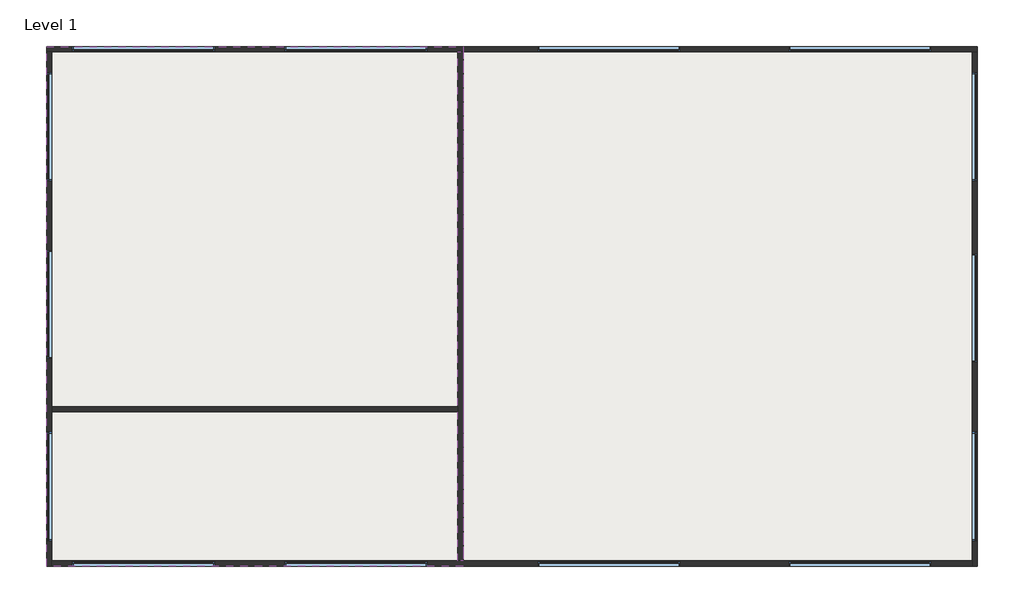
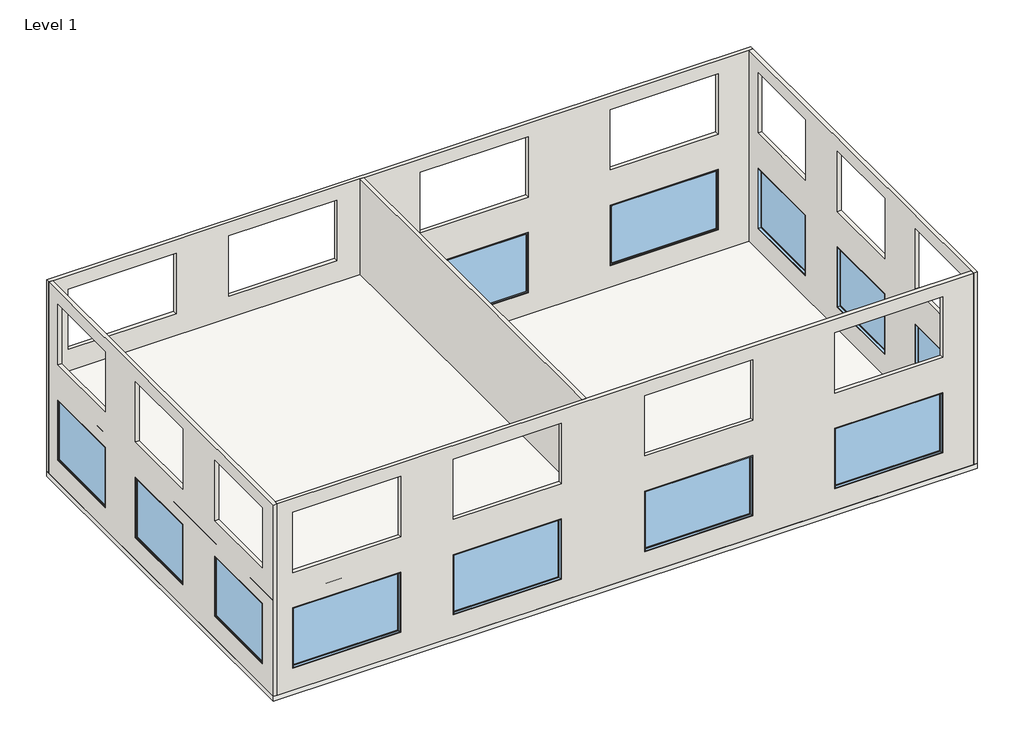
# One storey: 14 windows, 7 walls, 2 slabs.
"""IFC4 building model written with IfcOpenShell, lengths in millimetres."""

import ifcopenshell
import ifcopenshell.guid

model = None  # the IFC model being written
_history = None  # IfcOwnerHistory: only IFC2X3 demands one
_inside = {}  # id of a spatial element -> (the spatial element, [elements in it])
_under = {}  # id of a project, library or spatial element -> (it, [spatial elements below it])
_declared = {}  # id of a project -> (the project, [libraries it declares])
_typed = {}  # id of a type object -> (the type object, [elements of that type])
_made_of = {}  # id of a material, layer set ... -> (it, [elements and type objects made of it])


def new_model(schema):
    """Start an empty IFC model of exactly this schema.

    Asked for "IFC4X3", IfcOpenShell would pick the latest addendum, in which some entities
    have other attributes; the version numbers below select the first issue.
    IFC2X3 requires an IfcOwnerHistory on every rooted entity: one is made here for all.
    """
    global model, _history
    if schema == "IFC4X3":
        model = ifcopenshell.file(schema_version=(4, 3, 0, 0))
    else:
        model = ifcopenshell.file(schema=schema)
    _inside.clear()
    _under.clear()
    _declared.clear()
    _typed.clear()
    _made_of.clear()
    _history = None
    if model.schema == "IFC2X3":
        org = make("IfcOrganization", Name="unknown")
        user = make(
            "IfcPersonAndOrganization",
            ThePerson=make("IfcPerson", FamilyName="unknown"),
            TheOrganization=org,
        )
        app = make(
            "IfcApplication",
            ApplicationDeveloper=org,
            Version="unknown",
            ApplicationFullName="unknown",
            ApplicationIdentifier="unknown",
        )
        _history = make(
            "IfcOwnerHistory",
            OwningUser=user,
            OwningApplication=app,
            ChangeAction="ADDED",
            CreationDate=0,
        )
    return model


def make(cls, **values):
    """One entity of the class cls with the attributes given. An attribute that is None is left unset."""
    return model.create_entity(
        cls, **{name: value for name, value in values.items() if value is not None}
    )


def rooted(cls, **values):
    """An entity with a GlobalId (a new one), such as an element, a storey or a relation."""
    return make(cls, GlobalId=ifcopenshell.guid.new(), OwnerHistory=_history, **values)


def si_unit(unit_type, name, prefix=None):
    """IfcSIUnit, for example si_unit("LENGTHUNIT", "METRE", prefix="MILLI")."""
    return make("IfcSIUnit", UnitType=unit_type, Prefix=prefix, Name=name)


def assignment(units):
    """IfcUnitAssignment: the units of a project."""
    return None if units is None else make("IfcUnitAssignment", Units=units)


def point(xyz):
    """IfcCartesianPoint."""
    return None if xyz is None else make("IfcCartesianPoint", Coordinates=xyz)


def direction(xyz):
    """IfcDirection."""
    return None if xyz is None else make("IfcDirection", DirectionRatios=xyz)


def frame(location, z_axis=None, x_axis=None):
    """IfcAxis2Placement3D, a coordinate frame: its origin and axes. An axis left out is left unset."""
    return make(
        "IfcAxis2Placement3D",
        Location=point(location),
        Axis=direction(z_axis),
        RefDirection=direction(x_axis),
    )


def origin():
    """The frame at (0, 0, 0) with its axes left unset."""
    return frame((0.0, 0.0, 0.0))


def origin_with_axes():
    """The frame at (0, 0, 0) with the z axis (0, 0, 1) and the x axis (1, 0, 0) written out."""
    return frame((0.0, 0.0, 0.0), z_axis=(0.0, 0.0, 1.0), x_axis=(1.0, 0.0, 0.0))


def place(relative_to, where):
    """IfcLocalPlacement: puts the frame where relative to a parent placement (None: the world)."""
    return make(
        "IfcLocalPlacement", PlacementRelTo=relative_to, RelativePlacement=where
    )


def context(
    kind, dimensions, precision=None, world=None, true_north=None, identifier=None
):
    """IfcGeometricRepresentationContext, for example the 3D "Model" context."""
    return make(
        "IfcGeometricRepresentationContext",
        ContextIdentifier=identifier,
        ContextType=kind,
        CoordinateSpaceDimension=dimensions,
        Precision=precision,
        WorldCoordinateSystem=world,
        TrueNorth=true_north,
    )


def project(units=None, contexts=None):
    """IfcProject with its units and contexts."""
    return rooted(
        "IfcProject",
        Name="project",
        RepresentationContexts=contexts,
        UnitsInContext=assignment(units),
    )


def spatial(cls, under=None, at=None, **own):
    """A site, building, storey or space (cls), placed at a placement, below another one or the project."""
    s = rooted(cls, ObjectPlacement=at, **own)
    if under is not None:
        _under.setdefault(under.id(), (under, []))[1].append(s)
    return s


def polyline(points):
    """IfcPolyline through the points."""
    return make("IfcPolyline", Points=[point(p) for p in points])


def outline(outer, holes=None, kind="AREA"):
    """IfcArbitraryClosedProfileDef: a profile drawn as a closed curve; with holes, ...WithVoids."""
    if holes is None:
        return make("IfcArbitraryClosedProfileDef", ProfileType=kind, OuterCurve=outer)
    return make(
        "IfcArbitraryProfileDefWithVoids",
        ProfileType=kind,
        OuterCurve=outer,
        InnerCurves=holes,
    )


def extrude(swept, where, along, depth):
    """IfcExtrudedAreaSolid: the profile swept, set in the frame where, extruded along a direction by depth."""
    return make(
        "IfcExtrudedAreaSolid",
        SweptArea=swept,
        Position=where,
        ExtrudedDirection=direction(along),
        Depth=depth,
    )


def faces_of(points, faces, orient=None, outer=None):
    """IfcFace entities. A face is a list of loops; a loop is a list of indices into points, from 0.

    orient and outer hold one flag for each loop. By default every Orientation is true, the
    first loop of a face is its IfcFaceOuterBound and the others are IfcFaceBound.
    """
    made = []
    for i, loops in enumerate(faces):
        bounds = []
        for j, loop in enumerate(loops):
            is_outer = j == 0 if outer is None else outer[i][j]
            bounds.append(
                make(
                    "IfcFaceOuterBound" if is_outer else "IfcFaceBound",
                    Bound=make("IfcPolyLoop", Polygon=[points[k] for k in loop]),
                    Orientation=True if orient is None else orient[i][j],
                )
            )
        made.append(make("IfcFace", Bounds=bounds))
    return made


def faceted_brep(points, faces, orient=None, outer=None, voids=None):
    """IfcFacetedBrep: a solid bounded by flat faces; with voids (closed shells), ...WithVoids."""
    shared = [point(p) for p in points]
    hull = make("IfcClosedShell", CfsFaces=faces_of(shared, faces, orient, outer))
    if voids is None:
        return make("IfcFacetedBrep", Outer=hull)
    return make(
        "IfcFacetedBrepWithVoids",
        Outer=hull,
        Voids=[
            make(cls, CfsFaces=faces_of(shared, fs, o, b)) for cls, fs, o, b in voids
        ],
    )


def shape(context_of_items, identifier, shape_type, items):
    """IfcShapeRepresentation: the items that make up one representation, for example the "Body"."""
    return make(
        "IfcShapeRepresentation",
        ContextOfItems=context_of_items,
        RepresentationIdentifier=identifier,
        RepresentationType=shape_type,
        Items=items,
    )


def source(mapping_origin, context_of_items, identifier, shape_type, items):
    """IfcRepresentationMap: a shape defined once, which mapped items show again and again."""
    return make(
        "IfcRepresentationMap",
        MappingOrigin=mapping_origin,
        MappedRepresentation=shape(context_of_items, identifier, shape_type, items),
    )


def transform(
    local_origin,
    x_axis=None,
    y_axis=None,
    z_axis=None,
    scale=None,
    scale2=None,
    scale3=None,
    uniform=True,
):
    """IfcCartesianTransformationOperator3D, or its non-uniform kind. x_axis, y_axis, z_axis: its Axis1, 2, 3."""
    if uniform:
        return make(
            "IfcCartesianTransformationOperator3D",
            Axis1=direction(x_axis),
            Axis2=direction(y_axis),
            LocalOrigin=point(local_origin),
            Scale=scale,
            Axis3=direction(z_axis),
        )
    return make(
        "IfcCartesianTransformationOperator3DnonUniform",
        Axis1=direction(x_axis),
        Axis2=direction(y_axis),
        LocalOrigin=point(local_origin),
        Scale=scale,
        Axis3=direction(z_axis),
        Scale2=scale2,
        Scale3=scale3,
    )


def mapped(mapping_source, mapping_target):
    """IfcMappedItem: shows the shape of a source again, moved by a transform."""
    return make(
        "IfcMappedItem", MappingSource=mapping_source, MappingTarget=mapping_target
    )


def made_of(thing, what):
    """Note that an element or type object is made of a material, layer set ...; save() writes the relation."""
    if what is not None:
        _made_of.setdefault(what.id(), (what, []))[1].append(thing)
    return thing


def element(
    cls,
    number,
    at=None,
    inside=None,
    cuts=None,
    type_object=None,
    material=None,
    context=None,
    identifier="Body",
    shape_type=None,
    held_by="IfcProductDefinitionShape",
    body=None,
    shapes=None,
    **own,
):
    """One element of the class cls, such as IfcWall. Its Tag is "e" and its number.

    at: its placement. inside: the storey or other place that contains it. cuts: it is an
    opening in that element (IfcRelVoidsElement). A single representation is given by context,
    identifier, shape_type and body (its items); several are given by shapes. held_by: the class
    of the entity that holds the representations. save() writes the other relations.
    """
    e = rooted(cls, Tag="e%d" % number, ObjectPlacement=at, **own)
    if body is not None:
        shapes = [shape(context, identifier, shape_type, body)]
    if shapes is not None:
        e.Representation = make(held_by, Representations=shapes)
    if inside is not None:
        _inside.setdefault(inside.id(), (inside, []))[1].append(e)
    if cuts is not None:
        rooted(
            "IfcRelVoidsElement", RelatingBuildingElement=cuts, RelatedOpeningElement=e
        )
    if type_object is not None:
        _typed.setdefault(type_object.id(), (type_object, []))[1].append(e)
    return made_of(e, material)


def aggregate(whole, parts):
    """IfcRelAggregates: a whole, such as a stair, and the parts it consists of."""
    return rooted("IfcRelAggregates", RelatingObject=whole, RelatedObjects=parts)


def save(model, path):
    """Write the relations noted so far, then the file.

    IfcRelAggregates (storeys below a building ...), IfcRelContainedInSpatialStructure (elements
    in a storey), IfcRelDefinesByType, IfcRelAssociatesMaterial and IfcRelDeclares: one each for
    every whole, place, type object, material and project.
    """
    for whole, parts in _under.values():
        aggregate(whole, parts)
    for where, things in _inside.values():
        rooted(
            "IfcRelContainedInSpatialStructure",
            RelatedElements=things,
            RelatingStructure=where,
        )
    for kind, things in _typed.values():
        rooted("IfcRelDefinesByType", RelatedObjects=things, RelatingType=kind)
    for what, things in _made_of.values():
        rooted("IfcRelAssociatesMaterial", RelatedObjects=things, RelatingMaterial=what)
    for by, libraries in _declared.values():
        rooted("IfcRelDeclares", RelatingContext=by, RelatedDefinitions=libraries)
    model.write(path)


def m_fixed_2500x_4228mm_fd5e51e7(model_context):
    return source(origin(), model_context, "Body", "SweptSolid", [
        extrude(outline(polyline([(-2050.8, 54.2), (2050.8, 54.2), (2050.8, 42.2), (-2050.8, 42.2), (-2050.8, 54.2)])), frame((0.0, 0.0, 368.0), z_axis=(0.0, 0.0, 1.0), x_axis=(1.0, 0.0, 0.0)), (0.0, 0.0, 1.0), 2374.0),
        extrude(outline(polyline([(2786.0, -2094.8), (324.0, -2094.8), (324.0, 2094.8), (2786.0, 2094.8), (2786.0, -2094.8)]), holes=[polyline([(2742.0, -2050.8), (2742.0, 2050.8), (368.0, 2050.8), (368.0, -2050.8), (2742.0, -2050.8)])]), frame((0.0, 26.2, 0.0), z_axis=(0.0, 1.0, 0.0), x_axis=(0.0, 0.0, 1.0)), (0.0, 0.0, 1.0), 44.0),
        extrude(outline(polyline([(2805.0, -2113.8), (305.0, -2113.8), (305.0, 2113.8), (2805.0, 2113.8), (2805.0, -2113.8)]), holes=[polyline([(2786.0, -2094.8), (2786.0, 2094.8), (324.0, 2094.8), (324.0, -2094.8), (2786.0, -2094.8)])]), frame((0.0, 26.2, 0.0), z_axis=(0.0, 1.0, 0.0), x_axis=(0.0, 0.0, 1.0)), (0.0, 0.0, 1.0), 63.0),
        extrude(outline(polyline([(2805.0, -2113.8), (305.0, -2113.8), (305.0, 2113.8), (2805.0, 2113.8), (2805.0, -2113.8)]), holes=[polyline([(2773.0, -2081.8), (2773.0, 2081.8), (337.0, 2081.8), (337.0, -2081.8), (2773.0, -2081.8)])]), frame((0.0, -63.2, 0.0), z_axis=(0.0, 1.0, 0.0), x_axis=(0.0, 0.0, 1.0)), (0.0, 0.0, 1.0), 89.4),
    ])


def m_fixed_2500x_4228mm_f14c179f(model_context):
    return source(origin(), model_context, "Body", "SweptSolid", [
        extrude(outline(polyline([(-2050.8, -54.2), (-2050.8, -42.2), (2050.8, -42.2), (2050.8, -54.2), (-2050.8, -54.2)])), frame((0.0, 0.0, 368.0), z_axis=(0.0, 0.0, 1.0), x_axis=(1.0, 0.0, 0.0)), (0.0, 0.0, 1.0), 2374.0),
        extrude(outline(polyline([(2786.0, -2094.8), (324.0, -2094.8), (324.0, 2094.8), (2786.0, 2094.8), (2786.0, -2094.8)]), holes=[polyline([(2742.0, -2050.8), (2742.0, 2050.8), (368.0, 2050.8), (368.0, -2050.8), (2742.0, -2050.8)])]), frame((0.0, -70.2, 0.0), z_axis=(0.0, 1.0, 0.0), x_axis=(0.0, 0.0, 1.0)), (0.0, 0.0, 1.0), 44.0),
        extrude(outline(polyline([(2805.0, -2113.8), (305.0, -2113.8), (305.0, 2113.8), (2805.0, 2113.8), (2805.0, -2113.8)]), holes=[polyline([(2786.0, -2094.8), (2786.0, 2094.8), (324.0, 2094.8), (324.0, -2094.8), (2786.0, -2094.8)])]), frame((0.0, -89.2, 0.0), z_axis=(0.0, 1.0, 0.0), x_axis=(0.0, 0.0, 1.0)), (0.0, 0.0, 1.0), 63.0),
        extrude(outline(polyline([(2805.0, -2113.8), (305.0, -2113.8), (305.0, 2113.8), (2805.0, 2113.8), (2805.0, -2113.8)]), holes=[polyline([(2773.0, -2081.8), (2773.0, 2081.8), (337.0, 2081.8), (337.0, -2081.8), (2773.0, -2081.8)])]), frame((0.0, -26.2, 0.0), z_axis=(0.0, 1.0, 0.0), x_axis=(0.0, 0.0, 1.0)), (0.0, 0.0, 1.0), 89.4),
    ])


def m_fixed_2500x_3220mm_df94f4d0(model_context):
    return source(origin(), model_context, "Body", "SweptSolid", [
        extrude(outline(polyline([(-1546.8, 54.2), (1546.8, 54.2), (1546.8, 42.2), (-1546.8, 42.2), (-1546.8, 54.2)])), frame((0.0, 0.0, 368.0), z_axis=(0.0, 0.0, 1.0), x_axis=(1.0, 0.0, 0.0)), (0.0, 0.0, 1.0), 2374.0),
        extrude(outline(polyline([(2786.0, -1590.8), (324.0, -1590.8), (324.0, 1590.8), (2786.0, 1590.8), (2786.0, -1590.8)]), holes=[polyline([(2742.0, -1546.8), (2742.0, 1546.8), (368.0, 1546.8), (368.0, -1546.8), (2742.0, -1546.8)])]), frame((0.0, 26.2, 0.0), z_axis=(0.0, 1.0, 0.0), x_axis=(0.0, 0.0, 1.0)), (0.0, 0.0, 1.0), 44.0),
        extrude(outline(polyline([(2805.0, -1609.8), (305.0, -1609.8), (305.0, 1609.8), (2805.0, 1609.8), (2805.0, -1609.8)]), holes=[polyline([(2786.0, -1590.8), (2786.0, 1590.8), (324.0, 1590.8), (324.0, -1590.8), (2786.0, -1590.8)])]), frame((0.0, 26.2, 0.0), z_axis=(0.0, 1.0, 0.0), x_axis=(0.0, 0.0, 1.0)), (0.0, 0.0, 1.0), 63.0),
        extrude(outline(polyline([(2805.0, -1609.8), (305.0, -1609.8), (305.0, 1609.8), (2805.0, 1609.8), (2805.0, -1609.8)]), holes=[polyline([(2773.0, -1577.8), (2773.0, 1577.8), (337.0, 1577.8), (337.0, -1577.8), (2773.0, -1577.8)])]), frame((0.0, -63.2, 0.0), z_axis=(0.0, 1.0, 0.0), x_axis=(0.0, 0.0, 1.0)), (0.0, 0.0, 1.0), 89.4),
    ])


def m_fixed_2500x_3220mm_8b997f8c(model_context):
    return source(origin(), model_context, "Body", "SweptSolid", [
        extrude(outline(polyline([(-1546.8, -54.2), (-1546.8, -42.2), (1546.8, -42.2), (1546.8, -54.2), (-1546.8, -54.2)])), frame((0.0, 0.0, 368.0), z_axis=(0.0, 0.0, 1.0), x_axis=(1.0, 0.0, 0.0)), (0.0, 0.0, 1.0), 2374.0),
        extrude(outline(polyline([(2786.0, -1590.8), (324.0, -1590.8), (324.0, 1590.8), (2786.0, 1590.8), (2786.0, -1590.8)]), holes=[polyline([(2742.0, -1546.8), (2742.0, 1546.8), (368.0, 1546.8), (368.0, -1546.8), (2742.0, -1546.8)])]), frame((0.0, -70.2, 0.0), z_axis=(0.0, 1.0, 0.0), x_axis=(0.0, 0.0, 1.0)), (0.0, 0.0, 1.0), 44.0),
        extrude(outline(polyline([(2805.0, -1609.8), (305.0, -1609.8), (305.0, 1609.8), (2805.0, 1609.8), (2805.0, -1609.8)]), holes=[polyline([(2786.0, -1590.8), (2786.0, 1590.8), (324.0, 1590.8), (324.0, -1590.8), (2786.0, -1590.8)])]), frame((0.0, -89.2, 0.0), z_axis=(0.0, 1.0, 0.0), x_axis=(0.0, 0.0, 1.0)), (0.0, 0.0, 1.0), 63.0),
        extrude(outline(polyline([(2805.0, -1609.8), (305.0, -1609.8), (305.0, 1609.8), (2805.0, 1609.8), (2805.0, -1609.8)]), holes=[polyline([(2773.0, -1577.8), (2773.0, 1577.8), (337.0, 1577.8), (337.0, -1577.8), (2773.0, -1577.8)])]), frame((0.0, -26.2, 0.0), z_axis=(0.0, 1.0, 0.0), x_axis=(0.0, 0.0, 1.0)), (0.0, 0.0, 1.0), 89.4),
    ])


model = new_model("IFC4")

# Units and contexts
model_context = context("Model", 3, world=origin())
ifc_project = project(units=[si_unit("LENGTHUNIT", "METRE", prefix="MILLI")], contexts=[model_context])

# Site, building, storey
site = spatial("IfcSite", under=ifc_project)
building = spatial("IfcBuilding", under=site)
storey = spatial("IfcBuildingStorey", under=building, Name="Level 1", Elevation=0.0)

# Slabs
placement = place(None, origin())
element("IfcSlab", 1, ObjectType="160mm Concrete With 50mm Metal Deck", at=placement, inside=storey, context=model_context, shape_type="Brep", body=[
    faceted_brep([(29068.464681, 11296.9802217, -210.0), (29068.464681, -4095.4197783, -210.0), (1484.064681, -4095.4197783, -210.0), (1484.064681, 11296.9802217, -210.0), (29068.464681, 11296.9802217, 0.0), (1484.064681, 11296.9802217, 0.0), (1484.064681, -4095.4197783, 0.0), (28916.064681, -4095.4197783, 0.0), (29068.464681, -4095.4197783, 0.0), (29068.464681, 11144.5802217, 0.0)], [[[0, 1, 2, 3]], [[4, 5, 6, 7, 8, 9]], [[1, 0, 4, 9, 8]], [[2, 1, 8, 7, 6]], [[3, 2, 6, 5]], [[0, 3, 5, 4]]]),
])
element("IfcSlab", 2, ObjectType="160mm Concrete With 50mm Metal Deck", at=placement, inside=storey, context=model_context, shape_type="SweptSolid", body=[
    extrude(outline(polyline([(13828.464681, 11296.9802217), (13828.464681, -4095.4197783), (1484.064681, -4095.4197783), (1484.064681, 11296.9802217), (13828.464681, 11296.9802217)])), frame((0.0, 0.0, 3752.4), z_axis=(0.0, 0.0, 1.0), x_axis=(1.0, 0.0, 0.0)), (0.0, 0.0, 1.0), 210.0),
])

# Walls
element("IfcWall", 3, ObjectType="Generic - 152.4mm", at=placement, inside=storey, context=model_context, shape_type="Brep", body=[
    faceted_brep([(1484.064681, 11144.5802217, 0.0), (1636.464681, 11144.5802217, 0.0), (13676.064681, 11144.5802217, 0.0), (13828.464681, 11144.5802217, 0.0), (28916.064681, 11144.5802217, 0.0), (29068.464681, 11144.5802217, 0.0), (29068.464681, 11144.5802217, 7924.8), (28916.064681, 11144.5802217, 7924.8), (13828.464681, 11144.5802217, 7924.8), (13676.064681, 11144.5802217, 7924.8), (1636.464681, 11144.5802217, 7924.8), (1484.064681, 11144.5802217, 7924.8), (6474.064681, 11144.5802217, 902.4), (2246.464681, 11144.5802217, 902.4), (2246.464681, 11144.5802217, 3402.4), (6474.064681, 11144.5802217, 3402.4), (12766.064681, 11144.5802217, 902.4), (8538.464681, 11144.5802217, 902.4), (8538.464681, 11144.5802217, 3402.4), (12766.064681, 11144.5802217, 3402.4), (20266.064681, 11144.5802217, 902.4), (16038.464681, 11144.5802217, 902.4), (16038.464681, 11144.5802217, 3402.4), (20266.064681, 11144.5802217, 3402.4), (27706.064681, 11144.5802217, 902.4), (23478.464681, 11144.5802217, 902.4), (23478.464681, 11144.5802217, 3402.4), (27706.064681, 11144.5802217, 3402.4), (27706.064681, 11144.5802217, 4862.4), (23478.464681, 11144.5802217, 4862.4), (23478.464681, 11144.5802217, 7362.4), (27706.064681, 11144.5802217, 7362.4), (20266.064681, 11144.5802217, 4862.4), (16038.464681, 11144.5802217, 4862.4), (16038.464681, 11144.5802217, 7362.4), (20266.064681, 11144.5802217, 7362.4), (12766.064681, 11144.5802217, 4862.4), (8538.464681, 11144.5802217, 4862.4), (8538.464681, 11144.5802217, 7362.4), (12766.064681, 11144.5802217, 7362.4), (6474.064681, 11144.5802217, 4862.4), (2246.464681, 11144.5802217, 4862.4), (2246.464681, 11144.5802217, 7362.4), (6474.064681, 11144.5802217, 7362.4), (1484.064681, 11296.9802217, 0.0), (1484.064681, 11296.9802217, 7924.8), (29068.464681, 11296.9802217, 7924.8), (29068.464681, 11296.9802217, 0.0), (6474.064681, 11296.9802217, 902.4), (6474.064681, 11296.9802217, 3402.4), (2246.464681, 11296.9802217, 3402.4), (2246.464681, 11296.9802217, 902.4), (12766.064681, 11296.9802217, 902.4), (12766.064681, 11296.9802217, 3402.4), (8538.464681, 11296.9802217, 3402.4), (8538.464681, 11296.9802217, 902.4), (20266.064681, 11296.9802217, 902.4), (20266.064681, 11296.9802217, 3402.4), (16038.464681, 11296.9802217, 3402.4), (16038.464681, 11296.9802217, 902.4), (27706.064681, 11296.9802217, 902.4), (27706.064681, 11296.9802217, 3402.4), (23478.464681, 11296.9802217, 3402.4), (23478.464681, 11296.9802217, 902.4), (27706.064681, 11296.9802217, 4862.4), (27706.064681, 11296.9802217, 7362.4), (23478.464681, 11296.9802217, 7362.4), (23478.464681, 11296.9802217, 4862.4), (20266.064681, 11296.9802217, 4862.4), (20266.064681, 11296.9802217, 7362.4), (16038.464681, 11296.9802217, 7362.4), (16038.464681, 11296.9802217, 4862.4), (12766.064681, 11296.9802217, 4862.4), (12766.064681, 11296.9802217, 7362.4), (8538.464681, 11296.9802217, 7362.4), (8538.464681, 11296.9802217, 4862.4), (6474.064681, 11296.9802217, 4862.4), (6474.064681, 11296.9802217, 7362.4), (2246.464681, 11296.9802217, 7362.4), (2246.464681, 11296.9802217, 4862.4)], [[[0, 1, 2, 3, 4, 5, 6, 7, 8, 9, 10, 11], [12, 13, 14, 15], [16, 17, 18, 19], [20, 21, 22, 23], [24, 25, 26, 27], [28, 29, 30, 31], [32, 33, 34, 35], [36, 37, 38, 39], [40, 41, 42, 43]], [[44, 45, 46, 47], [48, 49, 50, 51], [52, 53, 54, 55], [56, 57, 58, 59], [60, 61, 62, 63], [64, 65, 66, 67], [68, 69, 70, 71], [72, 73, 74, 75], [76, 77, 78, 79]], [[5, 4, 3, 2, 1, 0, 44, 47]], [[11, 10, 9, 8, 7, 6, 46, 45]], [[6, 5, 47, 46]], [[0, 11, 45, 44]], [[49, 48, 12, 15]], [[50, 49, 15, 14]], [[51, 50, 14, 13]], [[48, 51, 13, 12]], [[53, 52, 16, 19]], [[54, 53, 19, 18]], [[55, 54, 18, 17]], [[52, 55, 17, 16]], [[57, 56, 20, 23]], [[58, 57, 23, 22]], [[59, 58, 22, 21]], [[56, 59, 21, 20]], [[61, 60, 24, 27]], [[62, 61, 27, 26]], [[63, 62, 26, 25]], [[60, 63, 25, 24]], [[65, 64, 28, 31]], [[66, 65, 31, 30]], [[67, 66, 30, 29]], [[64, 67, 29, 28]], [[69, 68, 32, 35]], [[70, 69, 35, 34]], [[71, 70, 34, 33]], [[68, 71, 33, 32]], [[73, 72, 36, 39]], [[74, 73, 39, 38]], [[75, 74, 38, 37]], [[72, 75, 37, 36]], [[77, 76, 40, 43]], [[78, 77, 43, 42]], [[79, 78, 42, 41]], [[76, 79, 41, 40]]]),
])
element("IfcWall", 4, ObjectType="Generic - 152.4mm", at=placement, inside=storey, context=model_context, shape_type="Brep", body=[
    faceted_brep([(28916.064681, 11144.5802217, 0.0), (28916.064681, -3943.0197783, 0.0), (28916.064681, -4095.4197783, 0.0), (28916.064681, -4095.4197783, 7924.8), (28916.064681, -3943.0197783, 7924.8), (28916.064681, 11144.5802217, 7924.8), (28916.064681, -3343.0197783, 902.4), (28916.064681, -123.4197783, 902.4), (28916.064681, -123.4197783, 3402.4), (28916.064681, -3343.0197783, 3402.4), (28916.064681, 1942.9802217, 902.4), (28916.064681, 5162.5802217, 902.4), (28916.064681, 5162.5802217, 3402.4), (28916.064681, 1942.9802217, 3402.4), (28916.064681, 7310.9802217, 902.4), (28916.064681, 10530.5802217, 902.4), (28916.064681, 10530.5802217, 3402.4), (28916.064681, 7310.9802217, 3402.4), (28916.064681, -3343.0197783, 4864.8), (28916.064681, -123.4197783, 4864.8), (28916.064681, -123.4197783, 7364.8), (28916.064681, -3343.0197783, 7364.8), (28916.064681, 1942.9802217, 4864.8), (28916.064681, 5162.5802217, 4864.8), (28916.064681, 5162.5802217, 7364.8), (28916.064681, 1942.9802217, 7364.8), (28916.064681, 7310.9802217, 4864.8), (28916.064681, 10530.5802217, 4864.8), (28916.064681, 10530.5802217, 7364.8), (28916.064681, 7310.9802217, 7364.8), (29068.464681, 11144.5802217, 0.0), (29068.464681, 11144.5802217, 7924.8), (29068.464681, -4095.4197783, 7924.8), (29068.464681, -4095.4197783, 0.0), (29068.464681, -3343.0197783, 902.4), (29068.464681, -3343.0197783, 3402.4), (29068.464681, -123.4197783, 3402.4), (29068.464681, -123.4197783, 902.4), (29068.464681, 1942.9802217, 902.4), (29068.464681, 1942.9802217, 3402.4), (29068.464681, 5162.5802217, 3402.4), (29068.464681, 5162.5802217, 902.4), (29068.464681, 7310.9802217, 902.4), (29068.464681, 7310.9802217, 3402.4), (29068.464681, 10530.5802217, 3402.4), (29068.464681, 10530.5802217, 902.4), (29068.464681, -3343.0197783, 4864.8), (29068.464681, -3343.0197783, 7364.8), (29068.464681, -123.4197783, 7364.8), (29068.464681, -123.4197783, 4864.8), (29068.464681, 1942.9802217, 4864.8), (29068.464681, 1942.9802217, 7364.8), (29068.464681, 5162.5802217, 7364.8), (29068.464681, 5162.5802217, 4864.8), (29068.464681, 7310.9802217, 4864.8), (29068.464681, 7310.9802217, 7364.8), (29068.464681, 10530.5802217, 7364.8), (29068.464681, 10530.5802217, 4864.8)], [[[0, 1, 2, 3, 4, 5], [6, 7, 8, 9], [10, 11, 12, 13], [14, 15, 16, 17], [18, 19, 20, 21], [22, 23, 24, 25], [26, 27, 28, 29]], [[30, 31, 32, 33], [34, 35, 36, 37], [38, 39, 40, 41], [42, 43, 44, 45], [46, 47, 48, 49], [50, 51, 52, 53], [54, 55, 56, 57]], [[2, 1, 0, 30, 33]], [[5, 4, 3, 32, 31]], [[0, 5, 31, 30]], [[35, 34, 6, 9]], [[36, 35, 9, 8]], [[37, 36, 8, 7]], [[34, 37, 7, 6]], [[39, 38, 10, 13]], [[40, 39, 13, 12]], [[41, 40, 12, 11]], [[38, 41, 11, 10]], [[43, 42, 14, 17]], [[44, 43, 17, 16]], [[45, 44, 16, 15]], [[42, 45, 15, 14]], [[3, 2, 33, 32]], [[47, 46, 18, 21]], [[48, 47, 21, 20]], [[49, 48, 20, 19]], [[46, 49, 19, 18]], [[51, 50, 22, 25]], [[52, 51, 25, 24]], [[53, 52, 24, 23]], [[50, 53, 23, 22]], [[55, 54, 26, 29]], [[56, 55, 29, 28]], [[57, 56, 28, 27]], [[54, 57, 27, 26]]]),
])
element("IfcWall", 5, ObjectType="Generic - 152.4mm", at=placement, inside=storey, context=model_context, shape_type="Brep", body=[
    faceted_brep([(28916.064681, -3943.0197783, 0.0), (13828.464681, -3943.0197783, 0.0), (13676.064681, -3943.0197783, 0.0), (1636.464681, -3943.0197783, 0.0), (1636.464681, -3943.0197783, 7924.8), (13676.064681, -3943.0197783, 7924.8), (13828.464681, -3943.0197783, 7924.8), (28916.064681, -3943.0197783, 7924.8), (27706.064681, -3943.0197783, 902.4), (27706.064681, -3943.0197783, 3402.4), (23478.464681, -3943.0197783, 3402.4), (23478.464681, -3943.0197783, 902.4), (20266.064681, -3943.0197783, 902.4), (20266.064681, -3943.0197783, 3402.4), (16038.464681, -3943.0197783, 3402.4), (16038.464681, -3943.0197783, 902.4), (12766.064681, -3943.0197783, 902.4), (12766.064681, -3943.0197783, 3402.4), (8538.464681, -3943.0197783, 3402.4), (8538.464681, -3943.0197783, 902.4), (6474.064681, -3943.0197783, 902.4), (6474.064681, -3943.0197783, 3402.4), (2246.464681, -3943.0197783, 3402.4), (2246.464681, -3943.0197783, 902.4), (27706.064681, -3943.0197783, 4862.4), (27706.064681, -3943.0197783, 7362.4), (23478.464681, -3943.0197783, 7362.4), (23478.464681, -3943.0197783, 4862.4), (20266.064681, -3943.0197783, 4862.4), (20266.064681, -3943.0197783, 7362.4), (16038.464681, -3943.0197783, 7362.4), (16038.464681, -3943.0197783, 4862.4), (12766.064681, -3943.0197783, 4862.4), (12766.064681, -3943.0197783, 7362.4), (8538.464681, -3943.0197783, 7362.4), (8538.464681, -3943.0197783, 4862.4), (6474.064681, -3943.0197783, 4862.4), (6474.064681, -3943.0197783, 7362.4), (2246.464681, -3943.0197783, 7362.4), (2246.464681, -3943.0197783, 4862.4), (28916.064681, -4095.4197783, 0.0), (28916.064681, -4095.4197783, 7924.8), (1636.464681, -4095.4197783, 7924.8), (1636.464681, -4095.4197783, 0.0), (27706.064681, -4095.4197783, 902.4), (23478.464681, -4095.4197783, 902.4), (23478.464681, -4095.4197783, 3402.4), (27706.064681, -4095.4197783, 3402.4), (20266.064681, -4095.4197783, 902.4), (16038.464681, -4095.4197783, 902.4), (16038.464681, -4095.4197783, 3402.4), (20266.064681, -4095.4197783, 3402.4), (12766.064681, -4095.4197783, 902.4), (8538.464681, -4095.4197783, 902.4), (8538.464681, -4095.4197783, 3402.4), (12766.064681, -4095.4197783, 3402.4), (6474.064681, -4095.4197783, 902.4), (2246.464681, -4095.4197783, 902.4), (2246.464681, -4095.4197783, 3402.4), (6474.064681, -4095.4197783, 3402.4), (27706.064681, -4095.4197783, 4862.4), (23478.464681, -4095.4197783, 4862.4), (23478.464681, -4095.4197783, 7362.4), (27706.064681, -4095.4197783, 7362.4), (20266.064681, -4095.4197783, 4862.4), (16038.464681, -4095.4197783, 4862.4), (16038.464681, -4095.4197783, 7362.4), (20266.064681, -4095.4197783, 7362.4), (12766.064681, -4095.4197783, 4862.4), (8538.464681, -4095.4197783, 4862.4), (8538.464681, -4095.4197783, 7362.4), (12766.064681, -4095.4197783, 7362.4), (6474.064681, -4095.4197783, 4862.4), (2246.464681, -4095.4197783, 4862.4), (2246.464681, -4095.4197783, 7362.4), (6474.064681, -4095.4197783, 7362.4)], [[[0, 1, 2, 3, 4, 5, 6, 7], [8, 9, 10, 11], [12, 13, 14, 15], [16, 17, 18, 19], [20, 21, 22, 23], [24, 25, 26, 27], [28, 29, 30, 31], [32, 33, 34, 35], [36, 37, 38, 39]], [[40, 41, 42, 43], [44, 45, 46, 47], [48, 49, 50, 51], [52, 53, 54, 55], [56, 57, 58, 59], [60, 61, 62, 63], [64, 65, 66, 67], [68, 69, 70, 71], [72, 73, 74, 75]], [[3, 2, 1, 0, 40, 43]], [[7, 6, 5, 4, 42, 41]], [[9, 8, 44, 47]], [[10, 9, 47, 46]], [[11, 10, 46, 45]], [[8, 11, 45, 44]], [[13, 12, 48, 51]], [[14, 13, 51, 50]], [[15, 14, 50, 49]], [[12, 15, 49, 48]], [[17, 16, 52, 55]], [[18, 17, 55, 54]], [[19, 18, 54, 53]], [[16, 19, 53, 52]], [[21, 20, 56, 59]], [[22, 21, 59, 58]], [[23, 22, 58, 57]], [[20, 23, 57, 56]], [[0, 7, 41, 40]], [[4, 3, 43, 42]], [[25, 24, 60, 63]], [[26, 25, 63, 62]], [[27, 26, 62, 61]], [[24, 27, 61, 60]], [[29, 28, 64, 67]], [[30, 29, 67, 66]], [[31, 30, 66, 65]], [[28, 31, 65, 64]], [[33, 32, 68, 71]], [[34, 33, 71, 70]], [[35, 34, 70, 69]], [[32, 35, 69, 68]], [[37, 36, 72, 75]], [[38, 37, 75, 74]], [[39, 38, 74, 73]], [[36, 39, 73, 72]]]),
])
element("IfcWall", 6, ObjectType="Generic - 152.4mm", at=placement, inside=storey, context=model_context, shape_type="Brep", body=[
    faceted_brep([(1636.464681, -4095.4197783, 0.0), (1636.464681, -3943.0197783, 0.0), (1636.464681, 476.5802217, 0.0), (1636.464681, 628.9802217, 0.0), (1636.464681, 11144.5802217, 0.0), (1636.464681, 11144.5802217, 7924.8), (1636.464681, -3943.0197783, 7924.8), (1636.464681, -4095.4197783, 7924.8), (1636.464681, 7310.9802217, 902.4), (1636.464681, 7310.9802217, 3402.4), (1636.464681, 10530.5802217, 3402.4), (1636.464681, 10530.5802217, 902.4), (1636.464681, 2042.9802217, 902.4), (1636.464681, 2042.9802217, 3402.4), (1636.464681, 5262.5802217, 3402.4), (1636.464681, 5262.5802217, 902.4), (1636.464681, -3343.0197783, 902.4), (1636.464681, -3343.0197783, 3402.4), (1636.464681, -123.4197783, 3402.4), (1636.464681, -123.4197783, 902.4), (1636.464681, -3343.0197783, 4864.8), (1636.464681, -3343.0197783, 7364.8), (1636.464681, -123.4197783, 7364.8), (1636.464681, -123.4197783, 4864.8), (1636.464681, 2042.9802217, 4864.8), (1636.464681, 2042.9802217, 7364.8), (1636.464681, 5262.5802217, 7364.8), (1636.464681, 5262.5802217, 4864.8), (1636.464681, 7310.9802217, 4864.8), (1636.464681, 7310.9802217, 7364.8), (1636.464681, 10530.5802217, 7364.8), (1636.464681, 10530.5802217, 4864.8), (1484.064681, -4095.4197783, 0.0), (1484.064681, -4095.4197783, 7924.8), (1484.064681, 11144.5802217, 7924.8), (1484.064681, 11144.5802217, 0.0), (1484.064681, 7310.9802217, 902.4), (1484.064681, 10530.5802217, 902.4), (1484.064681, 10530.5802217, 3402.4), (1484.064681, 7310.9802217, 3402.4), (1484.064681, 2042.9802217, 902.4), (1484.064681, 5262.5802217, 902.4), (1484.064681, 5262.5802217, 3402.4), (1484.064681, 2042.9802217, 3402.4), (1484.064681, -3343.0197783, 902.4), (1484.064681, -123.4197783, 902.4), (1484.064681, -123.4197783, 3402.4), (1484.064681, -3343.0197783, 3402.4), (1484.064681, -3343.0197783, 4864.8), (1484.064681, -123.4197783, 4864.8), (1484.064681, -123.4197783, 7364.8), (1484.064681, -3343.0197783, 7364.8), (1484.064681, 2042.9802217, 4864.8), (1484.064681, 5262.5802217, 4864.8), (1484.064681, 5262.5802217, 7364.8), (1484.064681, 2042.9802217, 7364.8), (1484.064681, 7310.9802217, 4864.8), (1484.064681, 10530.5802217, 4864.8), (1484.064681, 10530.5802217, 7364.8), (1484.064681, 7310.9802217, 7364.8)], [[[0, 1, 2, 3, 4, 5, 6, 7], [8, 9, 10, 11], [12, 13, 14, 15], [16, 17, 18, 19], [20, 21, 22, 23], [24, 25, 26, 27], [28, 29, 30, 31]], [[32, 33, 34, 35], [36, 37, 38, 39], [40, 41, 42, 43], [44, 45, 46, 47], [48, 49, 50, 51], [52, 53, 54, 55], [56, 57, 58, 59]], [[4, 3, 2, 1, 0, 32, 35]], [[7, 6, 5, 34, 33]], [[5, 4, 35, 34]], [[9, 8, 36, 39]], [[10, 9, 39, 38]], [[11, 10, 38, 37]], [[8, 11, 37, 36]], [[13, 12, 40, 43]], [[14, 13, 43, 42]], [[15, 14, 42, 41]], [[12, 15, 41, 40]], [[17, 16, 44, 47]], [[18, 17, 47, 46]], [[19, 18, 46, 45]], [[16, 19, 45, 44]], [[0, 7, 33, 32]], [[21, 20, 48, 51]], [[22, 21, 51, 50]], [[23, 22, 50, 49]], [[20, 23, 49, 48]], [[25, 24, 52, 55]], [[26, 25, 55, 54]], [[27, 26, 54, 53]], [[24, 27, 53, 52]], [[29, 28, 56, 59]], [[30, 29, 59, 58]], [[31, 30, 58, 57]], [[28, 31, 57, 56]]]),
])
element("IfcWall", 7, ObjectType="Generic - 152.4mm - Interior", at=placement, inside=storey, context=model_context, shape_type="Brep", body=[
    faceted_brep([(13828.464681, -3943.0197783, 0.0), (13828.464681, 11144.5802217, 0.0), (13828.464681, 11144.5802217, 3752.4), (13828.464681, -3943.0197783, 3752.4), (13676.064681, -3943.0197783, 0.0), (13676.064681, -3943.0197783, 3752.4), (13676.064681, 476.5802217, 3752.4), (13676.064681, 628.9802217, 3752.4), (13676.064681, 11144.5802217, 3752.4), (13676.064681, 11144.5802217, 0.0), (13676.064681, 628.9802217, 0.0), (13676.064681, 476.5802217, 0.0)], [[[0, 1, 2, 3]], [[4, 5, 6, 7, 8, 9, 10, 11]], [[1, 0, 4, 11, 10, 9]], [[0, 3, 5, 4]], [[2, 1, 9, 8]], [[3, 2, 8, 7, 6, 5]]]),
])
element("IfcWall", 8, ObjectType="Generic - 152.4mm - Interior", at=placement, inside=storey, context=model_context, shape_type="SweptSolid", body=[
    extrude(outline(polyline([(1636.464681, 628.9802217), (13676.064681, 628.9802217), (13676.064681, 476.5802217), (1636.464681, 476.5802217), (1636.464681, 628.9802217)])), origin_with_axes(), (0.0, 0.0, 1.0), 3752.4),
])
element("IfcWall", 9, ObjectType="Generic - 152.4mm - Interior", at=placement, inside=storey, context=model_context, shape_type="SweptSolid", body=[
    extrude(outline(polyline([(13676.064681, -3943.0197783), (13676.064681, 11144.5802217), (13828.464681, 11144.5802217), (13828.464681, -3943.0197783), (13676.064681, -3943.0197783)])), frame((0.0, 0.0, 3962.4), z_axis=(0.0, 0.0, 1.0), x_axis=(1.0, 0.0, 0.0)), (0.0, 0.0, 1.0), 3962.4),
])

# Windows
m_fixed_2500x_4228mm_shape = m_fixed_2500x_4228mm_fd5e51e7(model_context)
element("IfcWindow", 10, ObjectType="M_Fixed : 2500X 4228mm", at=placement, inside=storey, context=model_context, shape_type="MappedRepresentation", body=[
    mapped(m_fixed_2500x_4228mm_shape, transform((4360.264681, 11233.7802217, 597.4), x_axis=(-1.0, 0.0, 0.0), y_axis=(0.0, -1.0, 0.0), z_axis=(0.0, 0.0, 1.0))),
])
element("IfcWindow", 11, ObjectType="M_Fixed : 2500X 4228mm", at=placement, inside=storey, context=model_context, shape_type="MappedRepresentation", body=[
    mapped(m_fixed_2500x_4228mm_shape, transform((10652.264681, 11233.7802217, 597.4), x_axis=(-1.0, 0.0, 0.0), y_axis=(0.0, -1.0, 0.0), z_axis=(0.0, 0.0, 1.0))),
])
element("IfcWindow", 12, ObjectType="M_Fixed : 2500X 4228mm", at=placement, inside=storey, context=model_context, shape_type="MappedRepresentation", body=[
    mapped(m_fixed_2500x_4228mm_shape, transform((18152.264681, 11233.7802217, 597.4), x_axis=(-1.0, 0.0, 0.0), y_axis=(0.0, -1.0, 0.0), z_axis=(0.0, 0.0, 1.0))),
])
element("IfcWindow", 13, ObjectType="M_Fixed : 2500X 4228mm", at=placement, inside=storey, context=model_context, shape_type="MappedRepresentation", body=[
    mapped(m_fixed_2500x_4228mm_shape, transform((25592.264681, 11233.7802217, 597.4), x_axis=(-1.0, 0.0, 0.0), y_axis=(0.0, -1.0, 0.0), z_axis=(0.0, 0.0, 1.0))),
])
m_fixed_2500x_4228mm_2_shape = m_fixed_2500x_4228mm_f14c179f(model_context)
element("IfcWindow", 14, ObjectType="M_Fixed : 2500X 4228mm", at=placement, inside=storey, context=model_context, shape_type="MappedRepresentation", body=[
    mapped(m_fixed_2500x_4228mm_2_shape, transform((4360.264681, -4032.2197783, 597.4), x_axis=(-1.0, 0.0, 0.0), y_axis=(0.0, -1.0, 0.0), z_axis=(0.0, 0.0, 1.0))),
])
element("IfcWindow", 15, ObjectType="M_Fixed : 2500X 4228mm", at=placement, inside=storey, context=model_context, shape_type="MappedRepresentation", body=[
    mapped(m_fixed_2500x_4228mm_2_shape, transform((10652.264681, -4032.2197783, 597.4), x_axis=(-1.0, 0.0, 0.0), y_axis=(0.0, -1.0, 0.0), z_axis=(0.0, 0.0, 1.0))),
])
element("IfcWindow", 16, ObjectType="M_Fixed : 2500X 4228mm", at=placement, inside=storey, context=model_context, shape_type="MappedRepresentation", body=[
    mapped(m_fixed_2500x_4228mm_2_shape, transform((18152.264681, -4032.2197783, 597.4), x_axis=(-1.0, 0.0, 0.0), y_axis=(0.0, -1.0, 0.0), z_axis=(0.0, 0.0, 1.0))),
])
element("IfcWindow", 17, ObjectType="M_Fixed : 2500X 4228mm", at=placement, inside=storey, context=model_context, shape_type="MappedRepresentation", body=[
    mapped(m_fixed_2500x_4228mm_2_shape, transform((25592.264681, -4032.2197783, 597.4), x_axis=(-1.0, 0.0, 0.0), y_axis=(0.0, -1.0, 0.0), z_axis=(0.0, 0.0, 1.0))),
])
m_fixed_2500x_3220mm_shape = m_fixed_2500x_3220mm_df94f4d0(model_context)
element("IfcWindow", 18, ObjectType="M_Fixed : 2500x 3220mm", at=placement, inside=storey, context=model_context, shape_type="MappedRepresentation", body=[
    mapped(m_fixed_2500x_3220mm_shape, transform((1573.264681, 8920.7802217, 597.4), x_axis=(0.0, 1.0, 0.0), y_axis=(-1.0, 0.0, 0.0), z_axis=(0.0, 0.0, 1.0))),
])
element("IfcWindow", 19, ObjectType="M_Fixed : 2500x 3220mm", at=placement, inside=storey, context=model_context, shape_type="MappedRepresentation", body=[
    mapped(m_fixed_2500x_3220mm_shape, transform((1573.264681, 3652.7802217, 597.4), x_axis=(0.0, 1.0, 0.0), y_axis=(-1.0, 0.0, 0.0), z_axis=(0.0, 0.0, 1.0))),
])
element("IfcWindow", 20, ObjectType="M_Fixed : 2500x 3220mm", at=placement, inside=storey, context=model_context, shape_type="MappedRepresentation", body=[
    mapped(m_fixed_2500x_3220mm_shape, transform((1573.264681, -1733.2197783, 597.4), x_axis=(0.0, 1.0, 0.0), y_axis=(-1.0, 0.0, 0.0), z_axis=(0.0, 0.0, 1.0))),
])
m_fixed_2500x_3220mm_2_shape = m_fixed_2500x_3220mm_8b997f8c(model_context)
element("IfcWindow", 21, ObjectType="M_Fixed : 2500x 3220mm", at=placement, inside=storey, context=model_context, shape_type="MappedRepresentation", body=[
    mapped(m_fixed_2500x_3220mm_2_shape, transform((28979.264681, 8920.7802217, 597.4), x_axis=(0.0, 1.0, 0.0), y_axis=(-1.0, 0.0, 0.0), z_axis=(0.0, 0.0, 1.0))),
])
element("IfcWindow", 22, ObjectType="M_Fixed : 2500x 3220mm", at=placement, inside=storey, context=model_context, shape_type="MappedRepresentation", body=[
    mapped(m_fixed_2500x_3220mm_2_shape, transform((28979.264681, 3552.7802217, 597.4), x_axis=(0.0, 1.0, 0.0), y_axis=(-1.0, 0.0, 0.0), z_axis=(0.0, 0.0, 1.0))),
])
element("IfcWindow", 23, ObjectType="M_Fixed : 2500x 3220mm", at=placement, inside=storey, context=model_context, shape_type="MappedRepresentation", body=[
    mapped(m_fixed_2500x_3220mm_2_shape, transform((28979.264681, -1733.2197783, 597.4), x_axis=(0.0, 1.0, 0.0), y_axis=(-1.0, 0.0, 0.0), z_axis=(0.0, 0.0, 1.0))),
])

save(model, "model.ifc")

# Revit data of these elements
# Project information
#   Project Issue Date = "Issue Date"
#   Project Status = "Project Status"
#   Client Name = "Owner"
#   Project Address = "Enter address here"
#   Project Name = "Project Name"
#   Project Number = "Project Number"
# Type "160mm Concrete With 50mm Metal Deck"
#   Function = 0
#   Layers, outside or top first: 210 mm no material (function 1); 0 mm "Metal Deck" (function 200)
# Type "Generic - 152.4mm"
#   Layers, outside or top first: 152.4 mm no material (function 1)
# Type "Generic - 152.4mm - Interior"
#   Layers, outside or top first: 152.4 mm no material (function 1)
# Type "M_Fixed : 2500X 4228mm"
#   Type Mark = "25"
#   Height = 2500 mm
#   Default Sill Height = 305 mm
#   Width = 4227.6 mm
#   Window Inset = 19 mm
#   Frame Exterior Material = Sash
#   Frame Interior Material = Sash
#   Glass Pane Material = Glass
#   Sash = Sash
#   Wall Closure = (empty or 0)
# Type "M_Fixed : 2500x 3220mm"
#   Type Mark = "26"
#   Height = 2500 mm
#   Default Sill Height = 305 mm
#   Width = 3219.6 mm
#   Window Inset = 19 mm
#   Frame Exterior Material = Sash
#   Frame Interior Material = Sash
#   Glass Pane Material = Glass
#   Sash = Sash
#   Wall Closure = (empty or 0)
# Element 1 (IfcSlab, "160mm Concrete With 50mm Metal Deck")
#   Height Offset From Level = 0 mm
#   Phase Created = New Construction
#   Materials on its faces: "Metal Deck", "Default Floor"
# Element 2 (IfcSlab, "160mm Concrete With 50mm Metal Deck")
#   Height Offset From Level = 3962.4 mm
#   Phase Created = New Construction
#   Materials on its faces: "Metal Deck", "Default Floor"
# Elements 3, 4, 5, 6 (IfcWall, "Generic - 152.4mm")
#   Top Offset = 0 mm
#   Base Offset = 0 mm
#   wall height = 7924.8 mm
#   Phase Created = New Construction
#   Base Constraint = Level 1
#   Top Constraint = Roof Level
#   Materials on its faces: "Default Wall"
# Element 7 (IfcWall, "Generic - 152.4mm - Interior")
#   Top Offset = 3962.4 mm
#   Base Offset = 0 mm
#   wall height = 3752.4 mm
#   Phase Created = New Construction
#   Base Constraint = Level 1
#   Top Constraint = Level 1
#   Materials on its faces: "Default Wall"
# Element 8 (IfcWall, "Generic - 152.4mm - Interior")
#   Top Offset = 3862.4 mm
#   Base Offset = 0 mm
#   wall height = 3752.4 mm
#   Phase Created = New Construction
#   Base Constraint = Level 1
#   Top Constraint = Level 1
#   Materials on its faces: "Default Wall"
# Element 9 (IfcWall, "Generic - 152.4mm - Interior")
#   built-in parameter 1001111 = 3962.4 mm
#   Top Offset = 0 mm
#   Base Offset = 3962.4 mm
#   Unconnected Height = 3962.4 mm
#   wall height = 3962.4 mm
#   Phase Created = New Construction
#   Base Constraint = Level 1
#   Top Constraint = Roof Level
#   Materials on its faces: "Default Wall"
# Element 10 (IfcWindow, "M_Fixed : 2500X 4228mm")
#   Mark = "10"
#   Phase Created = New Construction
#   Materials on its faces: "Sash", "Glass"
# Element 11 (IfcWindow, "M_Fixed : 2500X 4228mm")
#   Mark = "11"
#   Phase Created = New Construction
#   Materials on its faces: "Sash", "Glass"
# Element 12 (IfcWindow, "M_Fixed : 2500X 4228mm")
#   Mark = "12"
#   Phase Created = New Construction
#   Materials on its faces: "Sash", "Glass"
# Element 13 (IfcWindow, "M_Fixed : 2500X 4228mm")
#   Mark = "13"
#   Phase Created = New Construction
#   Materials on its faces: "Sash", "Glass"
# Element 14 (IfcWindow, "M_Fixed : 2500X 4228mm")
#   Mark = "14"
#   Phase Created = New Construction
#   Materials on its faces: "Sash", "Glass"
# Element 15 (IfcWindow, "M_Fixed : 2500X 4228mm")
#   Mark = "15"
#   Phase Created = New Construction
#   Materials on its faces: "Sash", "Glass"
# Element 16 (IfcWindow, "M_Fixed : 2500X 4228mm")
#   Mark = "16"
#   Phase Created = New Construction
#   Materials on its faces: "Sash", "Glass"
# Element 17 (IfcWindow, "M_Fixed : 2500X 4228mm")
#   Mark = "17"
#   Phase Created = New Construction
#   Materials on its faces: "Sash", "Glass"
# Element 18 (IfcWindow, "M_Fixed : 2500x 3220mm")
#   Mark = "27"
#   Phase Created = New Construction
#   Materials on its faces: "Sash", "Glass"
# Element 19 (IfcWindow, "M_Fixed : 2500x 3220mm")
#   Mark = "28"
#   Phase Created = New Construction
#   Materials on its faces: "Sash", "Glass"
# Element 20 (IfcWindow, "M_Fixed : 2500x 3220mm")
#   Mark = "29"
#   Phase Created = New Construction
#   Materials on its faces: "Sash", "Glass"
# Element 21 (IfcWindow, "M_Fixed : 2500x 3220mm")
#   Mark = "30"
#   Phase Created = New Construction
#   Materials on its faces: "Sash", "Glass"
# Element 22 (IfcWindow, "M_Fixed : 2500x 3220mm")
#   Mark = "31"
#   Phase Created = New Construction
#   Materials on its faces: "Sash", "Glass"
# Element 23 (IfcWindow, "M_Fixed : 2500x 3220mm")
#   Mark = "32"
#   Phase Created = New Construction
#   Materials on its faces: "Sash", "Glass"
# Materials
#   "Metal Deck": class "Metal", colour RGB 247 247 247, transparency 0, Description = "Steel, mill finish", Cost = 0
#   "Sash": class "Wood", colour RGB 136 99 55, transparency 0
#   "Glass": class "Glass", colour RGB 0 128 192, transparency 0.9, Description = "Soda Lime Glass", Cost = 0
#   "Default Floor": class "Miscellaneous", colour RGB 127 127 127, transparency 0, Cost = 0
#   "Default Wall": class "Miscellaneous", colour RGB 128 128 128, transparency 0, Cost = 0
# Room at (7259.725, -1600.456) mm, phase "New Construction", upper level "Level 2", upper offset 0 mm, lower offset 0 mm
#   Number = "6"
#   Name = "Room"
# Room at (8198.725, 4816.984) mm, phase "New Construction", upper level "Level 2", upper offset 0 mm, lower offset 0 mm
#   Number = "7"
#   Name = "Room"
# Room at (21274.823, 2677.837) mm, phase "New Construction", upper level "Roof Level", upper offset 0 mm, lower offset 0 mm
#   Number = "8"
#   Name = "Room"
